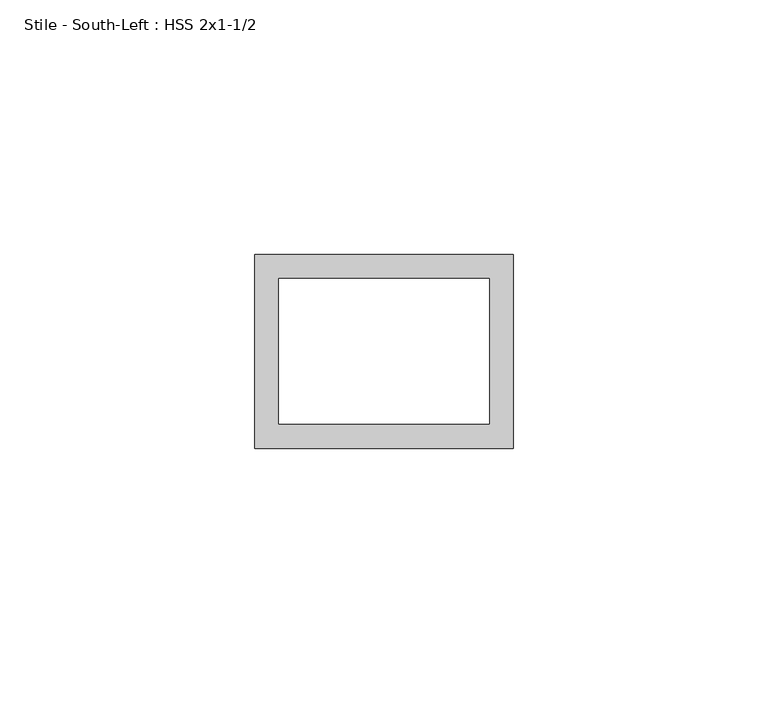
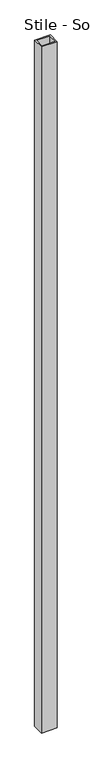
"""IFC4 building model written with IfcOpenShell, lengths in millimetres: proxy geometry, Stile - South-Left : HSS 2x1-1/2."""

from ifc_helpers import new_model, si_unit, frame, origin, place, context, project, spatial, polyline, outline, extrude, source, transform, mapped, element, save


def stile_south_left_hss_2x1_1_2_374c26f2(model_context):
    return source(origin(), model_context, "Body", "SweptSolid", [
        extrude(outline(polyline([(587365.8934739, -532883.8163841), (587416.6934739, -532883.8163841), (587416.6934739, -532921.9163841), (587365.8934739, -532921.9163841), (587365.8934739, -532883.8163841)]), holes=[polyline([(587370.6559739, -532888.5788841), (587370.6559739, -532917.1538841), (587411.9309739, -532917.1538841), (587411.9309739, -532888.5788841), (587370.6559739, -532888.5788841)])]), frame((0.0, 0.0, 50.8), z_axis=(0.0, 0.0, 1.0), x_axis=(1.0, 0.0, 0.0)), (0.0, 0.0, 1.0), 2349.5),
    ])


if __name__ == "__main__":
    model = new_model("IFC4")
    model_context = context("Model", 3, world=origin())
    ifc_project = project(units=[si_unit("LENGTHUNIT", "METRE", prefix="MILLI")], contexts=[model_context])
    site = spatial("IfcSite", under=ifc_project)
    building = spatial("IfcBuilding", under=site)
    placement = place(None, origin())
    stile_south_left_hss_2x1_1_2_shape = stile_south_left_hss_2x1_1_2_374c26f2(model_context)
    element("IfcBuildingElementProxy", 1, Name="Stile - South-Left : HSS 2x1-1/2", ObjectType="Stile - South-Left : HSS 2x1-1/2", at=placement, inside=building, context=model_context, shape_type="MappedRepresentation", body=[
        mapped(stile_south_left_hss_2x1_1_2_shape, transform((0.0, 0.0, 0.0), x_axis=(1.0, 0.0, 0.0), y_axis=(0.0, 1.0, 0.0), z_axis=(0.0, 0.0, 1.0))),
    ])
    save(model, "model.ifc")

# Revit data of these elements
# Element 1 (IfcBuildingElementProxy, "Stile - South-Left : HSS 2x1-1/2")
#   Materials on its faces: "1-1/2\"X2\" GALV. STL HSS TUBING"
# Materials
#   "1-1/2\"X2\" GALV. STL HSS TUBING": class "Generic", colour RGB 211 211 207, transparency 0, Cost = 0
